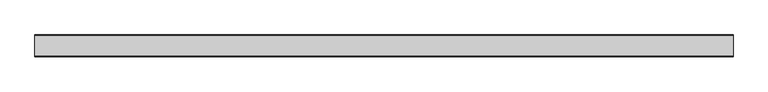
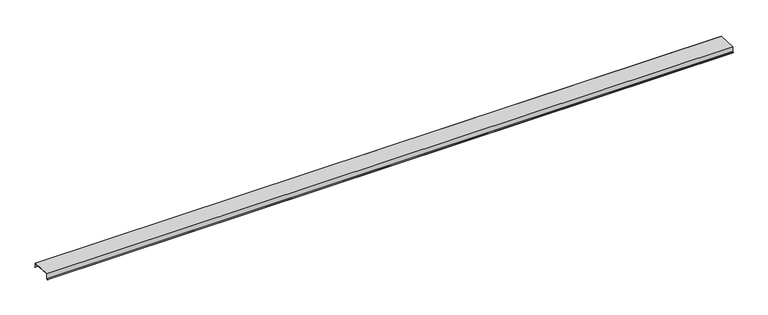
"""IFC4 building model written with IfcOpenShell, lengths in millimetres: proxy geometry, Generic Models 7:Generic Models 1:5:Generic Models 1:5 : Generic Models 7:Generic Models 1:337419:7 : Generic Models 7:Generic Models 1:5:Generic Models 1:5 : Generic Models 7:Generic Models 1:337419:311462."""

from ifc_helpers import new_model, si_unit, frame, origin, place, context, project, spatial, polyline, outline, extrude, source, transform, mapped, element, save


def generic_models_f82223a2(model_context):
    return source(origin(), model_context, "Body", "SweptSolid", [
        extrude(outline(polyline([(-579111.8163841, 6099.8348677), (-579111.8163841, 6188.1524863), (-578756.2163841, 6169.51628), (-578756.2163841, 6099.8348677), (-578743.5163841, 6087.1348677), (-578744.6389161, 6086.0123357), (-578757.8038841, 6099.1773037), (-578757.8038841, 6168.0097987), (-579110.2288841, 6186.4796103), (-579110.2288841, 6099.1773037), (-579123.3938521, 6086.0123357), (-579124.5163841, 6087.1348677), (-579111.8163841, 6099.8348677)])), frame((560646.6492239, 0.0, 0.0), z_axis=(1.0, 0.0, 0.0), x_axis=(0.0, 1.0, 0.0)), (0.0, 0.0, 1.0), 12250.7375001),
    ])


if __name__ == "__main__":
    model = new_model("IFC4")
    model_context = context("Model", 3, world=origin())
    ifc_project = project(units=[si_unit("LENGTHUNIT", "METRE", prefix="MILLI")], contexts=[model_context])
    site = spatial("IfcSite", under=ifc_project)
    building = spatial("IfcBuilding", under=site)
    placement = place(None, origin())
    generic_models_shape = generic_models_f82223a2(model_context)
    element("IfcBuildingElementProxy", 1, Name="Generic Models 7:Generic Models 1:5:Generic Models 1:5 : Generic Models 7:Generic Models 1:337419:7 : Generic Models 7:Generic Models 1:5:Generic Models 1:5 : Generic Models 7:Generic Models 1:337419:311462", ObjectType="Generic Models 7:Generic Models 1:5:Generic Models 1:5 : Generic Models 7:Generic Models 1:337419:7 : Generic Models 7:Generic Models 1:5:Generic Models 1:5 : Generic Models 7:Generic Models 1:337419:311462", at=placement, inside=building, context=model_context, shape_type="MappedRepresentation", body=[
        mapped(generic_models_shape, transform((0.0, 0.0, 0.0), x_axis=(1.0, 0.0, 0.0), y_axis=(0.0, 1.0, 0.0), z_axis=(0.0, 0.0, 1.0))),
    ])
    save(model, "model.ifc")

# Revit data of these elements
# Type "Generic Models 7:Generic Models 1:5:Generic Models 1:5 : Generic Models 7:Generic Models 1:337419:7 : Generic Models 7:Generic Models 1:5:Generic Models 1:5 : Generic Models 7:Generic Models 1:337419:311462"
#   NameOverride = "Generic Models 7:Generic Models 1:5:Generic Models 1:5 : Generic Models 7:Generic Models 1:337419:311462"
#   ObjectTypeOverride = "Generic Models 1:5 : Generic Models 7:Generic Models 1:337419"
#   Reference = "Generic Models 1"
#   Tag = "311462"
# Element 1 (IfcBuildingElementProxy, "Generic Models 7:Generic Models 1:5:Generic Models 1:5 : Generic Models 7:Generic Models 1:337419:7 : Generic Models 7:Generic Models 1:5:Generic Models 1:5 : Generic Models 7:Generic Models 1:337419:311462")
#   Materials on its faces: "SLOPED SHEET METAL COPING - (COLOR TO MATCH RESIN PANEL)"
# Materials
#   "SLOPED SHEET METAL COPING - (COLOR TO MATCH RESIN PANEL)": class "Generic", colour RGB 240 240 240, transparency 0, Keynote = "M07711300.01", Cost = 0
